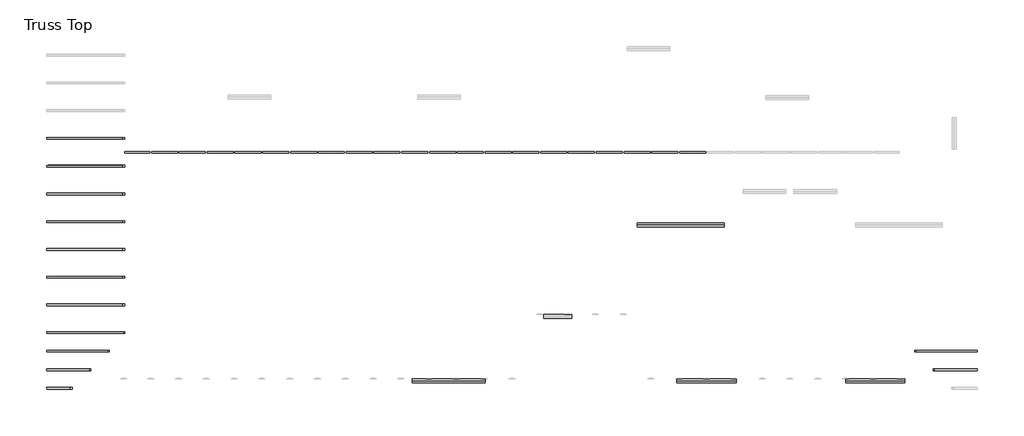
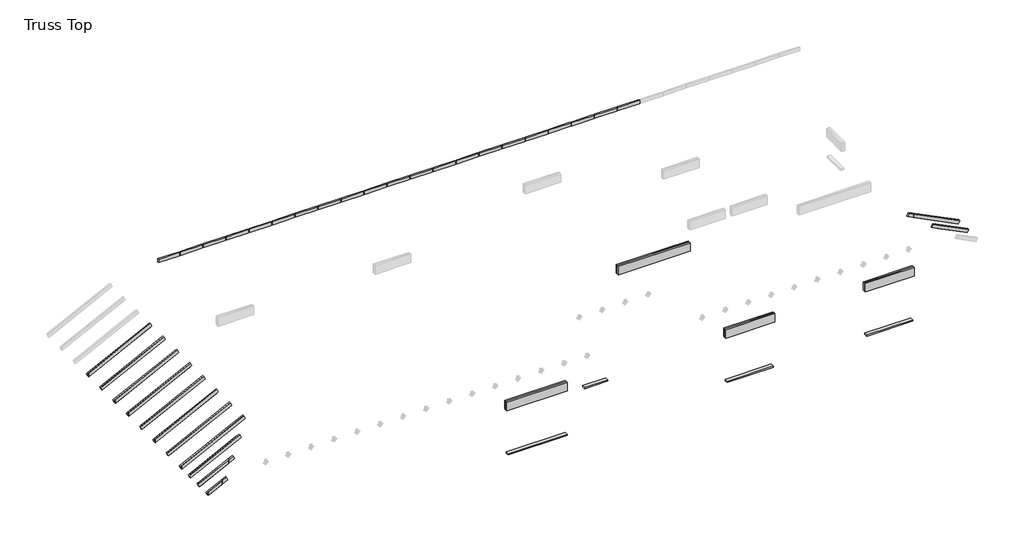
# One storey, part 1 of 3: 46 beams.
"""IFC4 building model written with IfcOpenShell, lengths in millimetres."""

import ifcopenshell
import ifcopenshell.guid

model = None  # the IFC model being written
_history = None  # IfcOwnerHistory: only IFC2X3 demands one
_inside = {}  # id of a spatial element -> (the spatial element, [elements in it])
_under = {}  # id of a project, library or spatial element -> (it, [spatial elements below it])
_declared = {}  # id of a project -> (the project, [libraries it declares])
_typed = {}  # id of a type object -> (the type object, [elements of that type])
_made_of = {}  # id of a material, layer set ... -> (it, [elements and type objects made of it])


def new_model(schema):
    """Start an empty IFC model of exactly this schema.

    Asked for "IFC4X3", IfcOpenShell would pick the latest addendum, in which some entities
    have other attributes; the version numbers below select the first issue.
    IFC2X3 requires an IfcOwnerHistory on every rooted entity: one is made here for all.
    """
    global model, _history
    if schema == "IFC4X3":
        model = ifcopenshell.file(schema_version=(4, 3, 0, 0))
    else:
        model = ifcopenshell.file(schema=schema)
    _inside.clear()
    _under.clear()
    _declared.clear()
    _typed.clear()
    _made_of.clear()
    _history = None
    if model.schema == "IFC2X3":
        org = make("IfcOrganization", Name="unknown")
        user = make(
            "IfcPersonAndOrganization",
            ThePerson=make("IfcPerson", FamilyName="unknown"),
            TheOrganization=org,
        )
        app = make(
            "IfcApplication",
            ApplicationDeveloper=org,
            Version="unknown",
            ApplicationFullName="unknown",
            ApplicationIdentifier="unknown",
        )
        _history = make(
            "IfcOwnerHistory",
            OwningUser=user,
            OwningApplication=app,
            ChangeAction="ADDED",
            CreationDate=0,
        )
    return model


def make(cls, **values):
    """One entity of the class cls with the attributes given. An attribute that is None is left unset."""
    return model.create_entity(
        cls, **{name: value for name, value in values.items() if value is not None}
    )


def rooted(cls, **values):
    """An entity with a GlobalId (a new one), such as an element, a storey or a relation."""
    return make(cls, GlobalId=ifcopenshell.guid.new(), OwnerHistory=_history, **values)


def si_unit(unit_type, name, prefix=None):
    """IfcSIUnit, for example si_unit("LENGTHUNIT", "METRE", prefix="MILLI")."""
    return make("IfcSIUnit", UnitType=unit_type, Prefix=prefix, Name=name)


def assignment(units):
    """IfcUnitAssignment: the units of a project."""
    return None if units is None else make("IfcUnitAssignment", Units=units)


def point(xyz):
    """IfcCartesianPoint."""
    return None if xyz is None else make("IfcCartesianPoint", Coordinates=xyz)


def direction(xyz):
    """IfcDirection."""
    return None if xyz is None else make("IfcDirection", DirectionRatios=xyz)


def frame(location, z_axis=None, x_axis=None):
    """IfcAxis2Placement3D, a coordinate frame: its origin and axes. An axis left out is left unset."""
    return make(
        "IfcAxis2Placement3D",
        Location=point(location),
        Axis=direction(z_axis),
        RefDirection=direction(x_axis),
    )


def origin():
    """The frame at (0, 0, 0) with its axes left unset."""
    return frame((0.0, 0.0, 0.0))


def place(relative_to, where):
    """IfcLocalPlacement: puts the frame where relative to a parent placement (None: the world)."""
    return make(
        "IfcLocalPlacement", PlacementRelTo=relative_to, RelativePlacement=where
    )


def context(
    kind, dimensions, precision=None, world=None, true_north=None, identifier=None
):
    """IfcGeometricRepresentationContext, for example the 3D "Model" context."""
    return make(
        "IfcGeometricRepresentationContext",
        ContextIdentifier=identifier,
        ContextType=kind,
        CoordinateSpaceDimension=dimensions,
        Precision=precision,
        WorldCoordinateSystem=world,
        TrueNorth=true_north,
    )


def project(units=None, contexts=None):
    """IfcProject with its units and contexts."""
    return rooted(
        "IfcProject",
        Name="project",
        RepresentationContexts=contexts,
        UnitsInContext=assignment(units),
    )


def spatial(cls, under=None, at=None, **own):
    """A site, building, storey or space (cls), placed at a placement, below another one or the project."""
    s = rooted(cls, ObjectPlacement=at, **own)
    if under is not None:
        _under.setdefault(under.id(), (under, []))[1].append(s)
    return s


def polyline(points):
    """IfcPolyline through the points."""
    return make("IfcPolyline", Points=[point(p) for p in points])


def outline(outer, holes=None, kind="AREA"):
    """IfcArbitraryClosedProfileDef: a profile drawn as a closed curve; with holes, ...WithVoids."""
    if holes is None:
        return make("IfcArbitraryClosedProfileDef", ProfileType=kind, OuterCurve=outer)
    return make(
        "IfcArbitraryProfileDefWithVoids",
        ProfileType=kind,
        OuterCurve=outer,
        InnerCurves=holes,
    )


def extrude(swept, where, along, depth):
    """IfcExtrudedAreaSolid: the profile swept, set in the frame where, extruded along a direction by depth."""
    return make(
        "IfcExtrudedAreaSolid",
        SweptArea=swept,
        Position=where,
        ExtrudedDirection=direction(along),
        Depth=depth,
    )


def faces_of(points, faces, orient=None, outer=None):
    """IfcFace entities. A face is a list of loops; a loop is a list of indices into points, from 0.

    orient and outer hold one flag for each loop. By default every Orientation is true, the
    first loop of a face is its IfcFaceOuterBound and the others are IfcFaceBound.
    """
    made = []
    for i, loops in enumerate(faces):
        bounds = []
        for j, loop in enumerate(loops):
            is_outer = j == 0 if outer is None else outer[i][j]
            bounds.append(
                make(
                    "IfcFaceOuterBound" if is_outer else "IfcFaceBound",
                    Bound=make("IfcPolyLoop", Polygon=[points[k] for k in loop]),
                    Orientation=True if orient is None else orient[i][j],
                )
            )
        made.append(make("IfcFace", Bounds=bounds))
    return made


def faceted_brep(points, faces, orient=None, outer=None, voids=None):
    """IfcFacetedBrep: a solid bounded by flat faces; with voids (closed shells), ...WithVoids."""
    shared = [point(p) for p in points]
    hull = make("IfcClosedShell", CfsFaces=faces_of(shared, faces, orient, outer))
    if voids is None:
        return make("IfcFacetedBrep", Outer=hull)
    return make(
        "IfcFacetedBrepWithVoids",
        Outer=hull,
        Voids=[
            make(cls, CfsFaces=faces_of(shared, fs, o, b)) for cls, fs, o, b in voids
        ],
    )


def shape(context_of_items, identifier, shape_type, items):
    """IfcShapeRepresentation: the items that make up one representation, for example the "Body"."""
    return make(
        "IfcShapeRepresentation",
        ContextOfItems=context_of_items,
        RepresentationIdentifier=identifier,
        RepresentationType=shape_type,
        Items=items,
    )


def source(mapping_origin, context_of_items, identifier, shape_type, items):
    """IfcRepresentationMap: a shape defined once, which mapped items show again and again."""
    return make(
        "IfcRepresentationMap",
        MappingOrigin=mapping_origin,
        MappedRepresentation=shape(context_of_items, identifier, shape_type, items),
    )


def transform(
    local_origin,
    x_axis=None,
    y_axis=None,
    z_axis=None,
    scale=None,
    scale2=None,
    scale3=None,
    uniform=True,
):
    """IfcCartesianTransformationOperator3D, or its non-uniform kind. x_axis, y_axis, z_axis: its Axis1, 2, 3."""
    if uniform:
        return make(
            "IfcCartesianTransformationOperator3D",
            Axis1=direction(x_axis),
            Axis2=direction(y_axis),
            LocalOrigin=point(local_origin),
            Scale=scale,
            Axis3=direction(z_axis),
        )
    return make(
        "IfcCartesianTransformationOperator3DnonUniform",
        Axis1=direction(x_axis),
        Axis2=direction(y_axis),
        LocalOrigin=point(local_origin),
        Scale=scale,
        Axis3=direction(z_axis),
        Scale2=scale2,
        Scale3=scale3,
    )


def mapped(mapping_source, mapping_target):
    """IfcMappedItem: shows the shape of a source again, moved by a transform."""
    return make(
        "IfcMappedItem", MappingSource=mapping_source, MappingTarget=mapping_target
    )


def made_of(thing, what):
    """Note that an element or type object is made of a material, layer set ...; save() writes the relation."""
    if what is not None:
        _made_of.setdefault(what.id(), (what, []))[1].append(thing)
    return thing


def element(
    cls,
    number,
    at=None,
    inside=None,
    cuts=None,
    type_object=None,
    material=None,
    context=None,
    identifier="Body",
    shape_type=None,
    held_by="IfcProductDefinitionShape",
    body=None,
    shapes=None,
    **own,
):
    """One element of the class cls, such as IfcWall. Its Tag is "e" and its number.

    at: its placement. inside: the storey or other place that contains it. cuts: it is an
    opening in that element (IfcRelVoidsElement). A single representation is given by context,
    identifier, shape_type and body (its items); several are given by shapes. held_by: the class
    of the entity that holds the representations. save() writes the other relations.
    """
    e = rooted(cls, Tag="e%d" % number, ObjectPlacement=at, **own)
    if body is not None:
        shapes = [shape(context, identifier, shape_type, body)]
    if shapes is not None:
        e.Representation = make(held_by, Representations=shapes)
    if inside is not None:
        _inside.setdefault(inside.id(), (inside, []))[1].append(e)
    if cuts is not None:
        rooted(
            "IfcRelVoidsElement", RelatingBuildingElement=cuts, RelatedOpeningElement=e
        )
    if type_object is not None:
        _typed.setdefault(type_object.id(), (type_object, []))[1].append(e)
    return made_of(e, material)


def aggregate(whole, parts):
    """IfcRelAggregates: a whole, such as a stair, and the parts it consists of."""
    return rooted("IfcRelAggregates", RelatingObject=whole, RelatedObjects=parts)


def save(model, path):
    """Write the relations noted so far, then the file.

    IfcRelAggregates (storeys below a building ...), IfcRelContainedInSpatialStructure (elements
    in a storey), IfcRelDefinesByType, IfcRelAssociatesMaterial and IfcRelDeclares: one each for
    every whole, place, type object, material and project.
    """
    for whole, parts in _under.values():
        aggregate(whole, parts)
    for where, things in _inside.values():
        rooted(
            "IfcRelContainedInSpatialStructure",
            RelatedElements=things,
            RelatingStructure=where,
        )
    for kind, things in _typed.values():
        rooted("IfcRelDefinesByType", RelatedObjects=things, RelatingType=kind)
    for what, things in _made_of.values():
        rooted("IfcRelAssociatesMaterial", RelatedObjects=things, RelatingMaterial=what)
    for by, libraries in _declared.values():
        rooted("IfcRelDeclares", RelatingContext=by, RelatedDefinitions=libraries)
    model.write(path)


def dimension_lumber_26660400(model_context):
    return source(origin(), model_context, "Body", "SweptSolid", [
        extrude(outline(polyline([(276.225, 19.05), (276.225, -19.05), (-276.225, -19.05), (-276.225, 19.05), (276.225, 19.05)])), frame((0.0, 0.0, -44.45), z_axis=(0.0, 0.0, 1.0), x_axis=(1.0, 0.0, 0.0)), (0.0, 0.0, 1.0), 88.9),
    ])


def dimension_lumber_d546034e(model_context):
    return source(origin(), model_context, "Body", "SweptSolid", [
        extrude(outline(polyline([(295.275, 19.05), (295.275, -19.05), (-276.225, -19.05), (-276.225, 19.05), (295.275, 19.05)])), frame((0.0, 0.0, -44.45), z_axis=(0.0, 0.0, 1.0), x_axis=(1.0, 0.0, 0.0)), (0.0, 0.0, 1.0), 88.9),
    ])


def dimension_lumber_37c2d9e3(model_context):
    return source(origin(), model_context, "Body", "SweptSolid", [
        extrude(outline(polyline([(609.5999994, 44.45), (609.5999994, -44.45), (-609.5999994, -44.45), (-609.5999994, 44.45), (609.5999994, 44.45)])), frame((0.0, 0.0, -19.05), z_axis=(0.0, 0.0, 1.0), x_axis=(1.0, 0.0, 0.0)), (0.0, 0.0, 1.0), 38.1),
    ])


def dimension_lumber_8e7dc767(model_context):
    return source(origin(), model_context, "Body", "SweptSolid", [
        extrude(outline(polyline([(790.5750003, 44.45), (790.5750003, -44.45), (-771.5249997, -44.45), (-771.5249997, 44.45), (790.5750003, 44.45)])), frame((0.0, 0.0, -19.05), z_axis=(0.0, 0.0, 1.0), x_axis=(1.0, 0.0, 0.0)), (0.0, 0.0, 1.0), 38.1),
    ])


def dimension_lumber_b6f9b94d(model_context):
    return source(origin(), model_context, "Body", "SweptSolid", [
        extrude(outline(polyline([(295.275, 44.45), (295.275, -44.45), (-314.3249994, -44.45), (-314.3249994, 44.45), (295.275, 44.45)])), frame((0.0, 0.0, -19.05), z_axis=(0.0, 0.0, 1.0), x_axis=(1.0, 0.0, 0.0)), (0.0, 0.0, 1.0), 38.1),
    ])


def dimension_lumber_2x10_header_exterior_8d927054(model_context):
    return source(origin(), model_context, "Body", "SweptSolid", [
        extrude(outline(polyline([(468.709375, 19.05), (468.709375, -19.05), (-826.690625, -19.05), (-826.690625, 19.05), (468.709375, 19.05)])), frame((0.0, 0.0, -117.475), z_axis=(0.0, 0.0, 1.0), x_axis=(1.0, 0.0, 0.0)), (0.0, 0.0, 1.0), 234.95),
    ])


def dimension_lumber_2x10_header_exterior_15155622(model_context):
    return source(origin(), model_context, "Body", "SweptSolid", [
        extrude(outline(polyline([(468.709375, 19.05), (468.709375, -19.05), (-1131.490625, -19.05), (-1131.490625, 19.05), (468.709375, 19.05)])), frame((0.0, 0.0, -117.475), z_axis=(0.0, 0.0, 1.0), x_axis=(1.0, 0.0, 0.0)), (0.0, 0.0, 1.0), 234.95),
    ])


def dimension_lumber_2x10_header_interior_91014728(model_context):
    return source(origin(), model_context, "Body", "SweptSolid", [
        extrude(outline(polyline([(468.709375, 19.05), (468.709375, -19.05), (-1434.7031244, -19.05), (-1434.7031244, 19.05), (468.709375, 19.05)])), frame((0.0, 0.0, -117.475), z_axis=(0.0, 0.0, 1.0), x_axis=(1.0, 0.0, 0.0)), (0.0, 0.0, 1.0), 234.95),
    ])


model = new_model("IFC4")

# Units and contexts
model_context = context("Model", 3, world=origin())
ifc_project = project(units=[si_unit("LENGTHUNIT", "METRE", prefix="MILLI")], contexts=[model_context])

# Site, building, storey
site = spatial("IfcSite", under=ifc_project)
building = spatial("IfcBuilding", under=site)
storey = spatial("IfcBuildingStorey", under=building, Name="Truss Top", Elevation=5452.4432216)

# Beams
placement = place(None, origin())
element("IfcBeam", 1, ObjectType="Dimension Lumber : Roof Lumbers", at=placement, inside=storey, context=model_context, shape_type="SweptSolid", body=[
    extrude(outline(polyline([(0.0, -38.1), (0.0, 0.0), (1874.2721787, 0.0), (1874.2721787, -38.1), (0.0, -38.1)])), frame((-6669.4579365, -4016.0040947, 2554.840297), z_axis=(-0.44721359549993367, 0.0, 0.8944271909999281), x_axis=(0.8944271909999281, 0.0, 0.44721359549993367)), (0.0, 0.0, 1.0), 88.9),
    extrude(outline(polyline([(2558.1548743, -6671.1152251), (2554.840297, -6669.4579365), (3393.040297, -4993.0579365), (3472.5548743, -5032.8152251), (2653.4048743, -6671.1152251), (2558.1548743, -6671.1152251)])), frame((0.0, -4054.1040947, 0.0), z_axis=(0.0, 1.0, 0.0), x_axis=(0.0, 0.0, 1.0)), (0.0, 0.0, 1.0), 38.1),
    extrude(outline(polyline([(2564.60625, -6649.9260305), (3393.040297, -4993.0579365), (3472.5548743, -5032.8152251), (2653.4048743, -6671.1152251), (2564.60625, -6671.1152251), (2564.60625, -6649.9260305)])), frame((0.0, -4054.1040947, 0.0), z_axis=(0.0, 1.0, 0.0), x_axis=(0.0, 0.0, 1.0)), (0.0, 0.0, 1.0), 38.1),
    extrude(outline(polyline([(2564.60625, -6649.9260305), (3373.1616527, -5032.8152251), (3472.5548743, -5032.8152251), (2653.4048743, -6671.1152251), (2564.60625, -6671.1152251), (2564.60625, -6649.9260305)])), frame((0.0, -4054.1040947, 0.0), z_axis=(0.0, 1.0, 0.0), x_axis=(0.0, 0.0, 1.0)), (0.0, 0.0, 1.0), 38.1),
])
element("IfcBeam", 2, ObjectType="Dimension Lumber : Roof Lumbers", at=placement, inside=storey, context=model_context, shape_type="SweptSolid", body=[
    extrude(outline(polyline([(0.0, -38.1), (0.0, 0.0), (1874.2721787, 0.0), (1874.2721787, -38.1), (0.0, -38.1)])), frame((-6669.4579365, -3406.4040947, 2554.840297), z_axis=(-0.4472135954999335, 0.0, 0.8944271909999282), x_axis=(0.8944271909999282, 0.0, 0.4472135954999335)), (0.0, 0.0, 1.0), 88.9),
    extrude(outline(polyline([(2558.1548743, -6671.1152251), (2554.840297, -6669.4579365), (3393.040297, -4993.0579365), (3472.5548743, -5032.8152251), (2653.4048743, -6671.1152251), (2558.1548743, -6671.1152251)])), frame((0.0, -3444.5040947, 0.0), z_axis=(0.0, 1.0, 0.0), x_axis=(0.0, 0.0, 1.0)), (0.0, 0.0, 1.0), 38.1),
    extrude(outline(polyline([(2564.60625, -6649.9260305), (3393.040297, -4993.0579365), (3472.5548743, -5032.8152251), (2653.4048743, -6671.1152251), (2564.60625, -6671.1152251), (2564.60625, -6649.9260305)])), frame((0.0, -3444.5040947, 0.0), z_axis=(0.0, 1.0, 0.0), x_axis=(0.0, 0.0, 1.0)), (0.0, 0.0, 1.0), 38.1),
    extrude(outline(polyline([(2564.60625, -6649.9260305), (3373.1616527, -5032.8152251), (3472.5548743, -5032.8152251), (2653.4048743, -6671.1152251), (2564.60625, -6671.1152251), (2564.60625, -6649.9260305)])), frame((0.0, -3444.5040947, 0.0), z_axis=(0.0, 1.0, 0.0), x_axis=(0.0, 0.0, 1.0)), (0.0, 0.0, 1.0), 38.1),
])
element("IfcBeam", 3, ObjectType="Dimension Lumber : Roof Lumbers", at=placement, inside=storey, context=model_context, shape_type="SweptSolid", body=[
    extrude(outline(polyline([(0.0, -38.1), (0.0, 0.0), (1874.2721787, 0.0), (1874.2721787, -38.1), (0.0, -38.1)])), frame((-6669.4579365, -2796.8040947, 2554.840297), z_axis=(-0.44721359549993367, 0.0, 0.8944271909999281), x_axis=(0.8944271909999281, 0.0, 0.44721359549993367)), (0.0, 0.0, 1.0), 88.9),
    extrude(outline(polyline([(2558.1548743, -6671.1152251), (2554.840297, -6669.4579365), (3393.040297, -4993.0579365), (3472.5548743, -5032.8152251), (2653.4048743, -6671.1152251), (2558.1548743, -6671.1152251)])), frame((0.0, -2834.9040947, 0.0), z_axis=(0.0, 1.0, 0.0), x_axis=(0.0, 0.0, 1.0)), (0.0, 0.0, 1.0), 38.1),
    extrude(outline(polyline([(2564.60625, -6649.9260305), (3393.040297, -4993.0579365), (3472.5548743, -5032.8152251), (2653.4048743, -6671.1152251), (2564.60625, -6671.1152251), (2564.60625, -6649.9260305)])), frame((0.0, -2834.9040947, 0.0), z_axis=(0.0, 1.0, 0.0), x_axis=(0.0, 0.0, 1.0)), (0.0, 0.0, 1.0), 38.1),
    extrude(outline(polyline([(2564.60625, -6649.9260305), (3373.1616527, -5032.8152251), (3472.5548743, -5032.8152251), (2653.4048743, -6671.1152251), (2564.60625, -6671.1152251), (2564.60625, -6649.9260305)])), frame((0.0, -2834.9040947, 0.0), z_axis=(0.0, 1.0, 0.0), x_axis=(0.0, 0.0, 1.0)), (0.0, 0.0, 1.0), 38.1),
])
element("IfcBeam", 4, ObjectType="Dimension Lumber : Roof Lumbers", at=placement, inside=storey, context=model_context, shape_type="SweptSolid", body=[
    extrude(outline(polyline([(0.0, -38.1), (0.0, 0.0), (1874.2721787, 0.0), (1874.2721787, -38.1), (0.0, -38.1)])), frame((-6669.4579365, -2187.2040947, 2554.840297), z_axis=(-0.44721359549993367, 0.0, 0.8944271909999281), x_axis=(0.8944271909999281, 0.0, 0.44721359549993367)), (0.0, 0.0, 1.0), 88.9),
    extrude(outline(polyline([(2558.1548743, -6671.1152251), (2554.840297, -6669.4579365), (3393.040297, -4993.0579365), (3472.5548743, -5032.8152251), (2653.4048743, -6671.1152251), (2558.1548743, -6671.1152251)])), frame((0.0, -2225.3040947, 0.0), z_axis=(0.0, 1.0, 0.0), x_axis=(0.0, 0.0, 1.0)), (0.0, 0.0, 1.0), 38.1),
    extrude(outline(polyline([(2564.60625, -6649.9260305), (3393.040297, -4993.0579365), (3472.5548743, -5032.8152251), (2653.4048743, -6671.1152251), (2564.60625, -6671.1152251), (2564.60625, -6649.9260305)])), frame((0.0, -2225.3040947, 0.0), z_axis=(0.0, 1.0, 0.0), x_axis=(0.0, 0.0, 1.0)), (0.0, 0.0, 1.0), 38.1),
    extrude(outline(polyline([(2564.60625, -6649.9260305), (3373.1616527, -5032.8152251), (3472.5548743, -5032.8152251), (2653.4048743, -6671.1152251), (2564.60625, -6671.1152251), (2564.60625, -6649.9260305)])), frame((0.0, -2225.3040947, 0.0), z_axis=(0.0, 1.0, 0.0), x_axis=(0.0, 0.0, 1.0)), (0.0, 0.0, 1.0), 38.1),
])
element("IfcBeam", 5, ObjectType="Dimension Lumber : Roof Lumbers", at=placement, inside=storey, context=model_context, shape_type="SweptSolid", body=[
    extrude(outline(polyline([(0.0, -38.1), (0.0, 0.0), (1874.2721787, 0.0), (1874.2721787, -38.1), (0.0, -38.1)])), frame((-6669.4579365, -968.0040947, 2554.840297), z_axis=(-0.44721359549993395, 0.0, 0.894427190999928), x_axis=(0.894427190999928, 0.0, 0.44721359549993395)), (0.0, 0.0, 1.0), 88.9),
    extrude(outline(polyline([(2558.1548743, -6671.1152251), (2554.840297, -6669.4579365), (3393.040297, -4993.0579365), (3472.5548743, -5032.8152251), (2653.4048743, -6671.1152251), (2558.1548743, -6671.1152251)])), frame((0.0, -1006.1040947, 0.0), z_axis=(0.0, 1.0, 0.0), x_axis=(0.0, 0.0, 1.0)), (0.0, 0.0, 1.0), 38.1),
    extrude(outline(polyline([(2564.60625, -6649.9260305), (3393.040297, -4993.0579365), (3472.5548743, -5032.8152251), (2653.4048743, -6671.1152251), (2564.60625, -6671.1152251), (2564.60625, -6649.9260305)])), frame((0.0, -1006.1040947, 0.0), z_axis=(0.0, 1.0, 0.0), x_axis=(0.0, 0.0, 1.0)), (0.0, 0.0, 1.0), 38.1),
    extrude(outline(polyline([(2564.60625, -6649.9260305), (3373.1616527, -5032.8152251), (3472.5548743, -5032.8152251), (2653.4048743, -6671.1152251), (2564.60625, -6671.1152251), (2564.60625, -6649.9260305)])), frame((0.0, -1006.1040947, 0.0), z_axis=(0.0, 1.0, 0.0), x_axis=(0.0, 0.0, 1.0)), (0.0, 0.0, 1.0), 38.1),
])
element("IfcBeam", 6, ObjectType="Dimension Lumber : Roof Lumbers", at=placement, inside=storey, context=model_context, shape_type="SweptSolid", body=[
    extrude(outline(polyline([(0.0, -38.1), (0.0, 0.0), (1874.2721787, 0.0), (1874.2721787, -38.1), (0.0, -38.1)])), frame((-6669.4579365, -358.4040947, 2554.840297), z_axis=(-0.4472135954999335, 0.0, 0.8944271909999282), x_axis=(0.8944271909999282, 0.0, 0.4472135954999335)), (0.0, 0.0, 1.0), 88.9),
    extrude(outline(polyline([(2558.1548743, -6671.1152251), (2554.840297, -6669.4579365), (3393.040297, -4993.0579365), (3472.5548743, -5032.8152251), (2653.4048743, -6671.1152251), (2558.1548743, -6671.1152251)])), frame((0.0, -396.5040947, 0.0), z_axis=(0.0, 1.0, 0.0), x_axis=(0.0, 0.0, 1.0)), (0.0, 0.0, 1.0), 38.1),
    extrude(outline(polyline([(2564.60625, -6649.9260305), (3393.040297, -4993.0579365), (3472.5548743, -5032.8152251), (2653.4048743, -6671.1152251), (2564.60625, -6671.1152251), (2564.60625, -6649.9260305)])), frame((0.0, -396.5040947, 0.0), z_axis=(0.0, 1.0, 0.0), x_axis=(0.0, 0.0, 1.0)), (0.0, 0.0, 1.0), 38.1),
    extrude(outline(polyline([(2564.60625, -6649.9260305), (3373.1616527, -5032.8152251), (3472.5548743, -5032.8152251), (2653.4048743, -6671.1152251), (2564.60625, -6671.1152251), (2564.60625, -6649.9260305)])), frame((0.0, -396.5040947, 0.0), z_axis=(0.0, 1.0, 0.0), x_axis=(0.0, 0.0, 1.0)), (0.0, 0.0, 1.0), 38.1),
])
element("IfcBeam", 7, ObjectType="Dimension Lumber : Roof Lumbers", at=placement, inside=storey, context=model_context, shape_type="SweptSolid", body=[
    extrude(outline(polyline([(0.0, -38.1), (0.0, 0.0), (1877.0701871, 0.0), (1877.0701871, -38.1), (0.0, -38.1)])), frame((-6669.4579365, -4625.6040947, 2554.840297), z_axis=(-0.4472135954999341, 0.0, 0.8944271909999277), x_axis=(0.8944271909999277, 0.0, 0.4472135954999341)), (0.0, 0.0, 1.0), 88.9),
    extrude(outline(polyline([(2558.1548743, -6671.1152251), (2554.840297, -6669.4579365), (3394.2916044, -4990.5553218), (3473.8061816, -5030.3126104), (2653.4048743, -6671.1152251), (2558.1548743, -6671.1152251)])), frame((0.0, -4663.7040947, 0.0), z_axis=(0.0, 1.0, 0.0), x_axis=(0.0, 0.0, 1.0)), (0.0, 0.0, 1.0), 38.1),
    extrude(outline(polyline([(2564.60625, -6649.9260305), (3394.2916044, -4990.5553218), (3473.8061816, -5030.3126104), (2653.4048743, -6671.1152251), (2564.60625, -6671.1152251), (2564.60625, -6649.9260305)])), frame((0.0, -4663.7040947, 0.0), z_axis=(0.0, 1.0, 0.0), x_axis=(0.0, 0.0, 1.0)), (0.0, 0.0, 1.0), 38.1),
    extrude(outline(polyline([(2564.60625, -6649.9260305), (3373.1616527, -5032.8152251), (3472.5548743, -5032.8152251), (2653.4048743, -6671.1152251), (2564.60625, -6671.1152251), (2564.60625, -6649.9260305)])), frame((0.0, -4663.7040947, 0.0), z_axis=(0.0, 1.0, 0.0), x_axis=(0.0, 0.0, 1.0)), (0.0, 0.0, 1.0), 38.1),
])
element("IfcBeam", 8, ObjectType="Dimension Lumber : Roof Lumbers", at=placement, inside=storey, context=model_context, shape_type="SweptSolid", body=[
    extrude(outline(polyline([(0.0, 38.1), (1874.2721787, 38.1), (1874.2721787, 0.0), (0.0, 0.0), (0.0, 38.1)])), frame((-6669.4579365, -1615.7040947, 2554.840297), z_axis=(-0.44721359549993367, 0.0, 0.8944271909999281), x_axis=(0.8944271909999281, 0.0, 0.44721359549993367)), (0.0, 0.0, 1.0), 88.9),
    extrude(outline(polyline([(2554.840297, -6669.4579365), (3393.040297, -4993.0579365), (3472.5548743, -5032.8152251), (2653.4048743, -6671.1152251), (2558.1548743, -6671.1152251), (2554.840297, -6669.4579365)])), frame((0.0, -1615.7040947, 0.0), z_axis=(0.0, 1.0, 0.0), x_axis=(0.0, 0.0, 1.0)), (0.0, 0.0, 1.0), 38.1),
    extrude(outline(polyline([(2564.60625, -6649.9260305), (3393.040297, -4993.0579365), (3472.5548743, -5032.8152251), (2653.4048743, -6671.1152251), (2564.60625, -6671.1152251), (2564.60625, -6649.9260305)])), frame((0.0, -1615.7040947, 0.0), z_axis=(0.0, 1.0, 0.0), x_axis=(0.0, 0.0, 1.0)), (0.0, 0.0, 1.0), 38.1),
    extrude(outline(polyline([(2564.60625, -6649.9260305), (3373.1616527, -5032.8152251), (3472.5548743, -5032.8152251), (2653.4048743, -6671.1152251), (2564.60625, -6671.1152251), (2564.60625, -6649.9260305)])), frame((0.0, -1615.7040947, 0.0), z_axis=(0.0, 1.0, 0.0), x_axis=(0.0, 0.0, 1.0)), (0.0, 0.0, 1.0), 38.1),
])
element("IfcBeam", 9, ObjectType="Dimension Lumber : Roof Lumbers", at=placement, inside=storey, context=model_context, shape_type="Brep", body=[
    faceted_brep([(-6709.2152251, -5070.1040947, 2634.3548743), (-6709.2152251, -5032.0040947, 2634.3548743), (-6669.4579365, -5032.0040947, 2554.840297), (-6669.4579365, -5070.1040947, 2554.840297), (-5368.8266367, -5070.1040947, 3304.5491685), (-5329.069348, -5070.1040947, 3225.0345912), (-5329.069348, -5032.0040947, 3225.0345912), (-5368.8266367, -5032.0040947, 3304.5491685)], [[[0, 1, 2, 3]], [[4, 5, 6, 7]], [[1, 0, 4, 7]], [[2, 1, 7, 6]], [[3, 2, 6, 5]], [[0, 3, 5, 4]]]),
    faceted_brep([(-6709.2152251, -5070.1040947, 2634.3548743), (-6709.2152251, -5032.0040947, 2634.3548743), (-6669.4579365, -5032.0040947, 2554.840297), (-6669.4579365, -5070.1040947, 2554.840297), (-5485.2059935, -5070.1040947, 3246.3594901), (-5447.1059935, -5032.0040947, 3265.4094901), (-5447.1059935, -5032.0040947, 3166.0162685), (-5485.2059935, -5070.1040947, 3146.9662685)], [[[0, 1, 2, 3]], [[1, 0, 4, 5]], [[2, 1, 5, 6]], [[3, 2, 6, 7]], [[0, 3, 7, 4]], [[5, 4, 7, 6]]]),
    faceted_brep([(-6709.2152251, -5070.1040947, 2634.3548743), (-6709.2152251, -5032.0040947, 2634.3548743), (-6674.340913, -5032.0040947, 2564.60625), (-6674.340913, -5070.1040947, 2564.60625), (-5485.2059935, -5070.1040947, 3246.3594901), (-5447.1059935, -5032.0040947, 3265.4094901), (-5447.1059935, -5032.0040947, 3166.0162685), (-6649.9260305, -5032.0040947, 2564.60625), (-6649.9260305, -5070.1040947, 2564.60625), (-5485.2059935, -5070.1040947, 3146.9662685)], [[[0, 1, 2, 3]], [[1, 0, 4, 5]], [[2, 1, 5, 6, 7]], [[0, 3, 8, 9, 4]], [[5, 4, 9, 6]], [[7, 6, 9, 8]], [[3, 2, 7, 8]]]),
    faceted_brep([(-6671.1152251, -5070.1040947, 2653.4048743), (-5485.2059935, -5070.1040947, 3246.3594901), (-5447.1059935, -5032.0040947, 3265.4094901), (-6671.1152251, -5032.0040947, 2653.4048743), (-6671.1152251, -5070.1040947, 2564.60625), (-6649.9260305, -5070.1040947, 2564.60625), (-5485.2059935, -5070.1040947, 3146.9662685), (-5447.1059935, -5032.0040947, 3166.0162685), (-6649.9260305, -5032.0040947, 2564.60625), (-6671.1152251, -5032.0040947, 2564.60625)], [[[0, 1, 2, 3]], [[4, 5, 6, 1, 0]], [[2, 1, 6, 7]], [[3, 2, 7, 8, 9]], [[8, 7, 6, 5]], [[9, 8, 5, 4]], [[0, 3, 9, 4]]]),
])
element("IfcBeam", 10, ObjectType="Dimension Lumber : Roof Lumbers", at=placement, inside=storey, context=model_context, shape_type="Brep", body=[
    faceted_brep([(-6709.2152251, -5476.5040947, 2634.3548743), (-6709.2152251, -5438.4040947, 2634.3548743), (-6669.4579365, -5438.4040947, 2554.840297), (-6669.4579365, -5476.5040947, 2554.840297), (-5777.7587484, -5476.5040947, 3100.0831127), (-5738.0014598, -5476.5040947, 3020.5685354), (-5738.0014598, -5438.4040947, 3020.5685354), (-5777.7587484, -5438.4040947, 3100.0831127)], [[[0, 1, 2, 3]], [[4, 5, 6, 7]], [[1, 0, 4, 7]], [[2, 1, 7, 6]], [[3, 2, 6, 5]], [[0, 3, 5, 4]]]),
    faceted_brep([(-6709.2152251, -5476.5040947, 2634.3548743), (-6709.2152251, -5438.4040947, 2634.3548743), (-6669.4579365, -5438.4040947, 2554.840297), (-6669.4579365, -5476.5040947, 2554.840297), (-5891.6059935, -5476.5040947, 3043.1594901), (-5853.5059935, -5438.4040947, 3062.2094901), (-5853.5059935, -5438.4040947, 2962.8162685), (-5891.6059935, -5476.5040947, 2943.7662685)], [[[0, 1, 2, 3]], [[1, 0, 4, 5]], [[2, 1, 5, 6]], [[3, 2, 6, 7]], [[0, 3, 7, 4]], [[5, 4, 7, 6]]]),
    faceted_brep([(-6709.2152251, -5476.5040947, 2634.3548743), (-6709.2152251, -5438.4040947, 2634.3548743), (-6674.340913, -5438.4040947, 2564.60625), (-6674.340913, -5476.5040947, 2564.60625), (-5891.6059935, -5476.5040947, 3043.1594901), (-5853.5059935, -5438.4040947, 3062.2094901), (-5853.5059935, -5438.4040947, 2962.8162685), (-6649.9260305, -5438.4040947, 2564.60625), (-6649.9260305, -5476.5040947, 2564.60625), (-5891.6059935, -5476.5040947, 2943.7662685)], [[[0, 1, 2, 3]], [[1, 0, 4, 5]], [[2, 1, 5, 6, 7]], [[0, 3, 8, 9, 4]], [[5, 4, 9, 6]], [[7, 6, 9, 8]], [[3, 2, 7, 8]]]),
    faceted_brep([(-6671.1152251, -5476.5040947, 2653.4048743), (-5891.6059935, -5476.5040947, 3043.1594901), (-5853.5059935, -5438.4040947, 3062.2094901), (-6671.1152251, -5438.4040947, 2653.4048743), (-6671.1152251, -5476.5040947, 2564.60625), (-6649.9260305, -5476.5040947, 2564.60625), (-5891.6059935, -5476.5040947, 2943.7662685), (-5853.5059935, -5438.4040947, 2962.8162685), (-6649.9260305, -5438.4040947, 2564.60625), (-6671.1152251, -5438.4040947, 2564.60625)], [[[0, 1, 2, 3]], [[4, 5, 6, 1, 0]], [[2, 1, 6, 7]], [[3, 2, 7, 8, 9]], [[8, 7, 6, 5]], [[9, 8, 5, 4]], [[0, 3, 9, 4]]]),
])
element("IfcBeam", 11, ObjectType="Dimension Lumber : Roof Lumbers", at=placement, inside=storey, context=model_context, shape_type="Brep", body=[
    faceted_brep([(-6709.2152251, -5882.9040947, 2634.3548743), (-6709.2152251, -5844.8040947, 2634.3548743), (-6669.4579365, -5844.8040947, 2554.840297), (-6669.4579365, -5882.9040947, 2554.840297), (-6186.6908601, -5882.9040947, 2895.6170568), (-6146.9335715, -5882.9040947, 2816.1024795), (-6146.9335715, -5844.8040947, 2816.1024795), (-6186.6908601, -5844.8040947, 2895.6170568)], [[[0, 1, 2, 3]], [[4, 5, 6, 7]], [[1, 0, 4, 7]], [[2, 1, 7, 6]], [[3, 2, 6, 5]], [[0, 3, 5, 4]]]),
    faceted_brep([(-6709.2152251, -5882.9040947, 2634.3548743), (-6709.2152251, -5844.8040947, 2634.3548743), (-6669.4579365, -5844.8040947, 2554.840297), (-6669.4579365, -5882.9040947, 2554.840297), (-6298.0059935, -5882.9040947, 2839.9594901), (-6259.9059935, -5844.8040947, 2859.0094901), (-6259.9059935, -5844.8040947, 2759.6162685), (-6298.0059935, -5882.9040947, 2740.5662685)], [[[0, 1, 2, 3]], [[1, 0, 4, 5]], [[2, 1, 5, 6]], [[3, 2, 6, 7]], [[0, 3, 7, 4]], [[5, 4, 7, 6]]]),
    faceted_brep([(-6709.2152251, -5882.9040947, 2634.3548743), (-6709.2152251, -5844.8040947, 2634.3548743), (-6674.340913, -5844.8040947, 2564.60625), (-6674.340913, -5882.9040947, 2564.60625), (-6298.0059935, -5882.9040947, 2839.9594901), (-6259.9059935, -5844.8040947, 2859.0094901), (-6259.9059935, -5844.8040947, 2759.6162685), (-6649.9260305, -5844.8040947, 2564.60625), (-6649.9260305, -5882.9040947, 2564.60625), (-6298.0059935, -5882.9040947, 2740.5662685)], [[[0, 1, 2, 3]], [[1, 0, 4, 5]], [[2, 1, 5, 6, 7]], [[0, 3, 8, 9, 4]], [[5, 4, 9, 6]], [[7, 6, 9, 8]], [[3, 2, 7, 8]]]),
    faceted_brep([(-6671.1152251, -5882.9040947, 2653.4048743), (-6298.0059935, -5882.9040947, 2839.9594901), (-6259.9059935, -5844.8040947, 2859.0094901), (-6671.1152251, -5844.8040947, 2653.4048743), (-6671.1152251, -5882.9040947, 2564.60625), (-6649.9260305, -5882.9040947, 2564.60625), (-6298.0059935, -5882.9040947, 2740.5662685), (-6259.9059935, -5844.8040947, 2759.6162685), (-6649.9260305, -5844.8040947, 2564.60625), (-6671.1152251, -5844.8040947, 2564.60625)], [[[0, 1, 2, 3]], [[4, 5, 6, 1, 0]], [[2, 1, 6, 7]], [[3, 2, 7, 8, 9]], [[8, 7, 6, 5]], [[9, 8, 5, 4]], [[0, 3, 9, 4]]]),
])
element("IfcBeam", 12, ObjectType="Dimension Lumber : Roof Lumbers", at=placement, inside=storey, context=model_context, shape_type="Brep", body=[
    faceted_brep([(13712.3847749, -5070.1040947, 2634.3548743), (13672.6274862, -5070.1040947, 2554.840297), (13672.6274862, -5032.0040947, 2554.840297), (13712.3847749, -5032.0040947, 2634.3548743), (12371.9961865, -5070.1040947, 3304.5491685), (12371.9961865, -5032.0040947, 3304.5491685), (12332.2388978, -5032.0040947, 3225.0345912), (12332.2388978, -5070.1040947, 3225.0345912)], [[[0, 1, 2, 3]], [[4, 5, 6, 7]], [[3, 5, 4, 0]], [[2, 6, 5, 3]], [[1, 7, 6, 2]], [[0, 4, 7, 1]]]),
    faceted_brep([(13712.3847749, -5070.1040947, 2634.3548743), (13672.6274862, -5070.1040947, 2554.840297), (13672.6274862, -5032.0040947, 2554.840297), (13712.3847749, -5032.0040947, 2634.3548743), (12488.3755432, -5070.1040947, 3246.3594901), (12488.3755432, -5070.1040947, 3146.9662685), (12450.2755432, -5032.0040947, 3166.0162685), (12450.2755432, -5032.0040947, 3265.4094901)], [[[0, 1, 2, 3]], [[0, 4, 5, 1]], [[1, 5, 6, 2]], [[2, 6, 7, 3]], [[3, 7, 4, 0]], [[4, 7, 6, 5]]]),
    faceted_brep([(13674.2847749, -5070.1040947, 2558.1548743), (13674.2847749, -5032.0040947, 2558.1548743), (13674.2847749, -5032.0040947, 2653.4048743), (13674.2847749, -5070.1040947, 2653.4048743), (13672.6274862, -5070.1040947, 2554.840297), (13672.6274862, -5032.0040947, 2554.840297), (12488.3755432, -5070.1040947, 3246.3594901), (12488.3755432, -5070.1040947, 3146.9662685), (12450.2755432, -5032.0040947, 3166.0162685), (12450.2755432, -5032.0040947, 3265.4094901)], [[[0, 1, 2, 3]], [[0, 4, 5, 1]], [[3, 6, 7, 4, 0]], [[4, 7, 8, 5]], [[5, 8, 9, 2, 1]], [[2, 9, 6, 3]], [[6, 9, 8, 7]]]),
])
element("IfcBeam", 13, ObjectType="Dimension Lumber : Roof Lumbers", at=placement, inside=storey, context=model_context, shape_type="Brep", body=[
    faceted_brep([(13712.3847749, -5476.5040947, 2634.3548743), (13672.6274862, -5476.5040947, 2554.840297), (13672.6274862, -5438.4040947, 2554.840297), (13712.3847749, -5438.4040947, 2634.3548743), (12780.9282982, -5476.5040947, 3100.0831127), (12780.9282982, -5438.4040947, 3100.0831127), (12741.1710095, -5438.4040947, 3020.5685354), (12741.1710095, -5476.5040947, 3020.5685354)], [[[0, 1, 2, 3]], [[4, 5, 6, 7]], [[3, 5, 4, 0]], [[2, 6, 5, 3]], [[1, 7, 6, 2]], [[0, 4, 7, 1]]]),
    faceted_brep([(13712.3847749, -5476.5040947, 2634.3548743), (13672.6274862, -5476.5040947, 2554.840297), (13672.6274862, -5438.4040947, 2554.840297), (13712.3847749, -5438.4040947, 2634.3548743), (12894.7755432, -5476.5040947, 3043.1594901), (12894.7755432, -5476.5040947, 2943.7662685), (12856.6755432, -5438.4040947, 2962.8162685), (12856.6755432, -5438.4040947, 3062.2094901)], [[[0, 1, 2, 3]], [[0, 4, 5, 1]], [[1, 5, 6, 2]], [[2, 6, 7, 3]], [[3, 7, 4, 0]], [[4, 7, 6, 5]]]),
    faceted_brep([(13674.2847749, -5476.5040947, 2558.1548743), (13674.2847749, -5438.4040947, 2558.1548743), (13674.2847749, -5438.4040947, 2653.4048743), (13674.2847749, -5476.5040947, 2653.4048743), (13672.6274862, -5476.5040947, 2554.840297), (13672.6274862, -5438.4040947, 2554.840297), (12894.7755432, -5476.5040947, 3043.1594901), (12894.7755432, -5476.5040947, 2943.7662685), (12856.6755432, -5438.4040947, 2962.8162685), (12856.6755432, -5438.4040947, 3062.2094901)], [[[0, 1, 2, 3]], [[0, 4, 5, 1]], [[3, 6, 7, 4, 0]], [[4, 7, 8, 5]], [[5, 8, 9, 2, 1]], [[2, 9, 6, 3]], [[6, 9, 8, 7]]]),
])
dimension_lumber_shape = dimension_lumber_26660400(model_context)
element("IfcBeam", 14, ObjectType="Dimension Lumber : Roof Lumbers", at=placement, inside=storey, context=model_context, shape_type="MappedRepresentation", body=[
    mapped(dimension_lumber_shape, transform((-4718.4902251, -682.2540947, 5399.6588466), x_axis=(-1.0, 0.0, 0.0), y_axis=(0.0, -1.0, 0.0), z_axis=(0.0, 0.0, 1.0))),
])
dimension_lumber_2_shape = dimension_lumber_d546034e(model_context)
element("IfcBeam", 15, ObjectType="Dimension Lumber : Roof Lumbers", at=placement, inside=storey, context=model_context, shape_type="MappedRepresentation", body=[
    mapped(dimension_lumber_2_shape, transform((7473.5097749, -682.2540947, 5399.6588466), x_axis=(-1.0, 0.0, 0.0), y_axis=(0.0, -1.0, 0.0), z_axis=(0.0, 0.0, 1.0))),
])
element("IfcBeam", 16, ObjectType="Dimension Lumber : Roof Lumbers", at=placement, inside=storey, context=model_context, shape_type="MappedRepresentation", body=[
    mapped(dimension_lumber_2_shape, transform((6863.9097749, -682.2540947, 5399.6588466), x_axis=(-1.0, 0.0, 0.0), y_axis=(0.0, -1.0, 0.0), z_axis=(0.0, 0.0, 1.0))),
])
element("IfcBeam", 17, ObjectType="Dimension Lumber : Roof Lumbers", at=placement, inside=storey, context=model_context, shape_type="MappedRepresentation", body=[
    mapped(dimension_lumber_2_shape, transform((6254.3097749, -682.2540947, 5399.6588466), x_axis=(-1.0, 0.0, 0.0), y_axis=(0.0, -1.0, 0.0), z_axis=(0.0, 0.0, 1.0))),
])
element("IfcBeam", 18, ObjectType="Dimension Lumber : Roof Lumbers", at=placement, inside=storey, context=model_context, shape_type="MappedRepresentation", body=[
    mapped(dimension_lumber_2_shape, transform((5644.7097749, -682.2540947, 5399.6588466), x_axis=(-1.0, 0.0, 0.0), y_axis=(0.0, -1.0, 0.0), z_axis=(0.0, 0.0, 1.0))),
])
element("IfcBeam", 19, ObjectType="Dimension Lumber : Roof Lumbers", at=placement, inside=storey, context=model_context, shape_type="MappedRepresentation", body=[
    mapped(dimension_lumber_2_shape, transform((5035.1097749, -682.2540947, 5399.6588466), x_axis=(-1.0, 0.0, 0.0), y_axis=(0.0, -1.0, 0.0), z_axis=(0.0, 0.0, 1.0))),
])
element("IfcBeam", 20, ObjectType="Dimension Lumber : Roof Lumbers", at=placement, inside=storey, context=model_context, shape_type="MappedRepresentation", body=[
    mapped(dimension_lumber_2_shape, transform((4425.5097749, -682.2540947, 5399.6588466), x_axis=(-1.0, 0.0, 0.0), y_axis=(0.0, -1.0, 0.0), z_axis=(0.0, 0.0, 1.0))),
])
element("IfcBeam", 21, ObjectType="Dimension Lumber : Roof Lumbers", at=placement, inside=storey, context=model_context, shape_type="MappedRepresentation", body=[
    mapped(dimension_lumber_2_shape, transform((3815.9097749, -682.2540947, 5399.6588466), x_axis=(-1.0, 0.0, 0.0), y_axis=(0.0, -1.0, 0.0), z_axis=(0.0, 0.0, 1.0))),
])
element("IfcBeam", 22, ObjectType="Dimension Lumber : Roof Lumbers", at=placement, inside=storey, context=model_context, shape_type="MappedRepresentation", body=[
    mapped(dimension_lumber_2_shape, transform((3206.3097749, -682.2540947, 5399.6588466), x_axis=(-1.0, 0.0, 0.0), y_axis=(0.0, -1.0, 0.0), z_axis=(0.0, 0.0, 1.0))),
])
element("IfcBeam", 23, ObjectType="Dimension Lumber : Roof Lumbers", at=placement, inside=storey, context=model_context, shape_type="MappedRepresentation", body=[
    mapped(dimension_lumber_2_shape, transform((2596.7097749, -682.2540947, 5399.6588466), x_axis=(-1.0, 0.0, 0.0), y_axis=(0.0, -1.0, 0.0), z_axis=(0.0, 0.0, 1.0))),
])
element("IfcBeam", 24, ObjectType="Dimension Lumber : Roof Lumbers", at=placement, inside=storey, context=model_context, shape_type="MappedRepresentation", body=[
    mapped(dimension_lumber_2_shape, transform((1987.1097749, -682.2540947, 5399.6588466), x_axis=(-1.0, 0.0, 0.0), y_axis=(0.0, -1.0, 0.0), z_axis=(0.0, 0.0, 1.0))),
])
element("IfcBeam", 25, ObjectType="Dimension Lumber : Roof Lumbers", at=placement, inside=storey, context=model_context, shape_type="MappedRepresentation", body=[
    mapped(dimension_lumber_2_shape, transform((1377.5097749, -682.2540947, 5399.6588466), x_axis=(-1.0, 0.0, 0.0), y_axis=(0.0, -1.0, 0.0), z_axis=(0.0, 0.0, 1.0))),
])
element("IfcBeam", 26, ObjectType="Dimension Lumber : Roof Lumbers", at=placement, inside=storey, context=model_context, shape_type="MappedRepresentation", body=[
    mapped(dimension_lumber_2_shape, transform((767.9097749, -682.2540947, 5399.6588466), x_axis=(-1.0, 0.0, 0.0), y_axis=(0.0, -1.0, 0.0), z_axis=(0.0, 0.0, 1.0))),
])
element("IfcBeam", 27, ObjectType="Dimension Lumber : Roof Lumbers", at=placement, inside=storey, context=model_context, shape_type="MappedRepresentation", body=[
    mapped(dimension_lumber_2_shape, transform((158.3097749, -682.2540947, 5399.6588466), x_axis=(-1.0, 0.0, 0.0), y_axis=(0.0, -1.0, 0.0), z_axis=(0.0, 0.0, 1.0))),
])
element("IfcBeam", 28, ObjectType="Dimension Lumber : Roof Lumbers", at=placement, inside=storey, context=model_context, shape_type="MappedRepresentation", body=[
    mapped(dimension_lumber_2_shape, transform((-451.2902251, -682.2540947, 5399.6588466), x_axis=(-1.0, 0.0, 0.0), y_axis=(0.0, -1.0, 0.0), z_axis=(0.0, 0.0, 1.0))),
])
element("IfcBeam", 29, ObjectType="Dimension Lumber : Roof Lumbers", at=placement, inside=storey, context=model_context, shape_type="MappedRepresentation", body=[
    mapped(dimension_lumber_2_shape, transform((-1060.8902251, -682.2540947, 5399.6588466), x_axis=(-1.0, 0.0, 0.0), y_axis=(0.0, -1.0, 0.0), z_axis=(0.0, 0.0, 1.0))),
])
element("IfcBeam", 30, ObjectType="Dimension Lumber : Roof Lumbers", at=placement, inside=storey, context=model_context, shape_type="MappedRepresentation", body=[
    mapped(dimension_lumber_2_shape, transform((-1670.4902251, -682.2540947, 5399.6588466), x_axis=(-1.0, 0.0, 0.0), y_axis=(0.0, -1.0, 0.0), z_axis=(0.0, 0.0, 1.0))),
])
element("IfcBeam", 31, ObjectType="Dimension Lumber : Roof Lumbers", at=placement, inside=storey, context=model_context, shape_type="MappedRepresentation", body=[
    mapped(dimension_lumber_2_shape, transform((-2280.0902251, -682.2540947, 5399.6588466), x_axis=(-1.0, 0.0, 0.0), y_axis=(0.0, -1.0, 0.0), z_axis=(0.0, 0.0, 1.0))),
])
element("IfcBeam", 32, ObjectType="Dimension Lumber : Roof Lumbers", at=placement, inside=storey, context=model_context, shape_type="MappedRepresentation", body=[
    mapped(dimension_lumber_2_shape, transform((-2889.6902251, -682.2540947, 5399.6588466), x_axis=(-1.0, 0.0, 0.0), y_axis=(0.0, -1.0, 0.0), z_axis=(0.0, 0.0, 1.0))),
])
element("IfcBeam", 33, ObjectType="Dimension Lumber : Roof Lumbers", at=placement, inside=storey, context=model_context, shape_type="MappedRepresentation", body=[
    mapped(dimension_lumber_2_shape, transform((-3499.2902251, -682.2540947, 5399.6588466), x_axis=(-1.0, 0.0, 0.0), y_axis=(0.0, -1.0, 0.0), z_axis=(0.0, 0.0, 1.0))),
])
element("IfcBeam", 34, ObjectType="Dimension Lumber : Roof Lumbers", at=placement, inside=storey, context=model_context, shape_type="MappedRepresentation", body=[
    mapped(dimension_lumber_2_shape, transform((-4108.8902251, -682.2540947, 5399.6588466), x_axis=(-1.0, 0.0, 0.0), y_axis=(0.0, -1.0, 0.0), z_axis=(0.0, 0.0, 1.0))),
])
dimension_lumber_3_shape = dimension_lumber_37c2d9e3(model_context)
element("IfcBeam", 35, ObjectType="Dimension Lumber : Opening Plate 2*4 Exterior", at=placement, inside=storey, context=model_context, shape_type="MappedRepresentation", body=[
    mapped(dimension_lumber_3_shape, transform((11466.0722749, -5705.1040947, 817.959375), x_axis=(1.0, 0.0, 0.0), y_axis=(0.0, 1.0, 0.0), z_axis=(0.0, 0.0, 1.0))),
])
element("IfcBeam", 36, ObjectType="Dimension Lumber : Opening Plate 2*4 Exterior", at=placement, inside=storey, context=model_context, shape_type="MappedRepresentation", body=[
    mapped(dimension_lumber_3_shape, transform((7768.7847755, -5705.1040947, 817.959375), x_axis=(1.0, 0.0, 0.0), y_axis=(0.0, 1.0, 0.0), z_axis=(0.0, 0.0, 1.0))),
])
dimension_lumber_4_shape = dimension_lumber_8e7dc767(model_context)
element("IfcBeam", 37, ObjectType="Dimension Lumber : Opening Plate 2*4 Exterior", at=placement, inside=storey, context=model_context, shape_type="MappedRepresentation", body=[
    mapped(dimension_lumber_4_shape, transform((2126.8097746, -5705.1040947, 817.959375), x_axis=(1.0, 0.0, 0.0), y_axis=(0.0, 1.0, 0.0), z_axis=(0.0, 0.0, 1.0))),
])
dimension_lumber_5_shape = dimension_lumber_b6f9b94d(model_context)
element("IfcBeam", 38, ObjectType="Dimension Lumber : Opening Plate 2*4 Exterior", at=placement, inside=storey, context=model_context, shape_type="MappedRepresentation", body=[
    mapped(dimension_lumber_5_shape, transform((4517.4097749, -4282.7040947, 817.959375), x_axis=(1.0, 0.0, 0.0), y_axis=(0.0, 1.0, 0.0), z_axis=(0.0, 0.0, 1.0))),
])
dimension_lumber_2x10_header_exterior_shape = dimension_lumber_2x10_header_exterior_8d927054(model_context)
element("IfcBeam", 39, ObjectType="Dimension Lumber : 2x10 Header Exterior", at=placement, inside=storey, context=model_context, shape_type="MappedRepresentation", body=[
    mapped(dimension_lumber_2x10_header_exterior_shape, transform((11287.0816499, -5730.5040947, 2173.684375), x_axis=(-1.0, 0.0, 0.0), y_axis=(0.0, -1.0, 0.0), z_axis=(0.0, 0.0, 1.0))),
])
element("IfcBeam", 40, ObjectType="Dimension Lumber : 2x10 Header Exterior", at=placement, inside=storey, context=model_context, shape_type="MappedRepresentation", body=[
    mapped(dimension_lumber_2x10_header_exterior_shape, transform((11287.0816499, -5679.7040947, 2173.684375), x_axis=(-1.0, 0.0, 0.0), y_axis=(0.0, -1.0, 0.0), z_axis=(0.0, 0.0, 1.0))),
])
element("IfcBeam", 41, ObjectType="Dimension Lumber : 2x10 Header Exterior", at=placement, inside=storey, context=model_context, shape_type="MappedRepresentation", body=[
    mapped(dimension_lumber_2x10_header_exterior_shape, transform((7589.7941505, -5730.5040947, 2173.684375), x_axis=(-1.0, 0.0, 0.0), y_axis=(0.0, -1.0, 0.0), z_axis=(0.0, 0.0, 1.0))),
])
element("IfcBeam", 42, ObjectType="Dimension Lumber : 2x10 Header Exterior", at=placement, inside=storey, context=model_context, shape_type="MappedRepresentation", body=[
    mapped(dimension_lumber_2x10_header_exterior_shape, transform((7589.7941505, -5679.7040947, 2173.684375), x_axis=(-1.0, 0.0, 0.0), y_axis=(0.0, -1.0, 0.0), z_axis=(0.0, 0.0, 1.0))),
])
dimension_lumber_2x10_header_exterior_2_shape = dimension_lumber_2x10_header_exterior_15155622(model_context)
element("IfcBeam", 43, ObjectType="Dimension Lumber : 2x10 Header Exterior", at=placement, inside=storey, context=model_context, shape_type="MappedRepresentation", body=[
    mapped(dimension_lumber_2x10_header_exterior_2_shape, transform((1785.8941493, -5730.5040947, 2173.684375), x_axis=(-1.0, 0.0, 0.0), y_axis=(0.0, -1.0, 0.0), z_axis=(0.0, 0.0, 1.0))),
])
element("IfcBeam", 44, ObjectType="Dimension Lumber : 2x10 Header Exterior", at=placement, inside=storey, context=model_context, shape_type="MappedRepresentation", body=[
    mapped(dimension_lumber_2x10_header_exterior_2_shape, transform((1785.8941493, -5679.7040947, 2173.684375), x_axis=(-1.0, 0.0, 0.0), y_axis=(0.0, -1.0, 0.0), z_axis=(0.0, 0.0, 1.0))),
])
dimension_lumber_2x10_header_interior_shape = dimension_lumber_2x10_header_interior_91014728(model_context)
element("IfcBeam", 45, ObjectType="Dimension Lumber : 2x10 Header Interior", at=placement, inside=storey, context=model_context, shape_type="MappedRepresentation", body=[
    mapped(dimension_lumber_2x10_header_interior_shape, transform((6719.8441505, -2301.5040947, 2173.684375), x_axis=(-1.0, 0.0, 0.0), y_axis=(0.0, -1.0, 0.0), z_axis=(0.0, 0.0, 1.0))),
])
element("IfcBeam", 46, ObjectType="Dimension Lumber : 2x10 Header Interior", at=placement, inside=storey, context=model_context, shape_type="MappedRepresentation", body=[
    mapped(dimension_lumber_2x10_header_interior_shape, transform((6719.8441505, -2250.7040947, 2173.684375), x_axis=(-1.0, 0.0, 0.0), y_axis=(0.0, -1.0, 0.0), z_axis=(0.0, 0.0, 1.0))),
])

save(model, "model.ifc")

# Revit data of these elements
# Type "Dimension Lumber : Roof Lumbers"
#   Assembly Code = "B10"
#   A = 0.0364583 SF
#   Length [instance default] = 5' - 0"
#   b = 0' - 1 1/2"
#   d = 0' - 3 1/2"
#   Structural Material [instance default] = Softwood, Lumber
# Type "Dimension Lumber : Opening Plate 2*4 Exterior"
#   Assembly Code = "B10"
#   A = 0.0364583 SF
#   Length [instance default] = 5' - 0"
#   b = 0' - 3 1/2"
#   d = 0' - 1 1/2"
#   Structural Material [instance default] = Softwood, Lumber
# Type "Dimension Lumber : 2x10 Header Exterior"
#   Assembly Code = "B10"
#   A = 0.0963889 SF
#   Length [instance default] = 5' - 0"
#   b = 0' - 1 1/2"
#   d = 0' - 9 1/4"
#   Structural Material [instance default] = Softwood, Lumber
# Type "Dimension Lumber : 2x10 Header Interior"
#   Assembly Code = "B10"
#   A = 0.0963889 SF
#   Length [instance default] = 5' - 0"
#   b = 0' - 1 1/2"
#   d = 0' - 9 1/4"
#   Structural Material [instance default] = Softwood, Lumber
# Elements 1, 2, 3, 4, 5, 6, 7, 8, 14, 15, 16, 17, 18, 19, 20, 21, 22, 23, 24, 25, 26, 27, 28, 29, 30, 31, 32, 33, 34 (IfcBeam, "Dimension Lumber : Roof Lumbers")
#   Structural Material = Douglas Fir #2
#   Phase Created = New Construction
#   Materials on its faces: "Douglas Fir #2"
# Elements 9, 10, 11, 12, 13 (IfcBeam, "Dimension Lumber : Roof Lumbers")
#   Structural Material = Softwood, Lumber
#   Phase Created = New Construction
#   Materials on its faces: "Softwood, Lumber"
# Elements 35, 36, 37, 38 (IfcBeam, "Dimension Lumber : Opening Plate 2*4 Exterior")
#   Structural Material = Douglas Fir #2
#   Phase Created = New Construction
#   Materials on its faces: "Douglas Fir #2"
# Elements 39, 40, 41, 42, 43, 44 (IfcBeam, "Dimension Lumber : 2x10 Header Exterior")
#   Comments = ""
#   Structural Material = Douglas Fir #2
#   Phase Created = New Construction
#   Materials on its faces: "Douglas Fir #2"
# Elements 45, 46 (IfcBeam, "Dimension Lumber : 2x10 Header Interior")
#   Comments = ""
#   Structural Material = Douglas Fir #2
#   Phase Created = New Construction
#   Materials on its faces: "Douglas Fir #2"
# Materials
#   "Softwood, Lumber": class "Wood", colour RGB 223 192 134, transparency 0, Description = "Pinus Echinata", Cost = 0
#   "Douglas Fir #2": class "Wood", colour RGB 223 192 134, transparency 0, Description = "Pinus Echinata", Cost = 0
